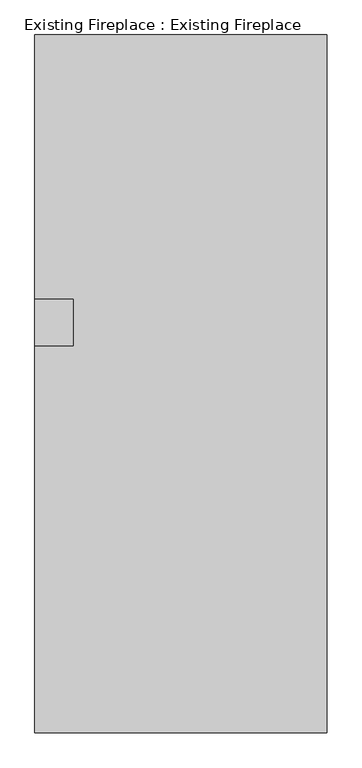
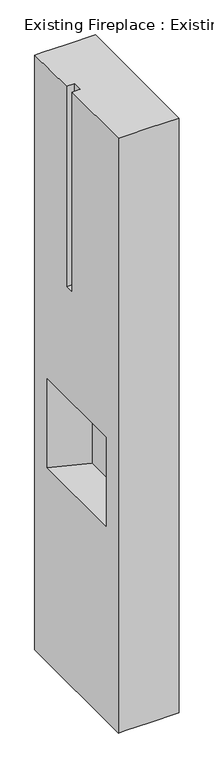
"""IFC4 building model written with IfcOpenShell, lengths in millimetres: proxy geometry, Existing Fireplace : Existing Fireplace."""

import ifcopenshell
import ifcopenshell.guid

model = None  # the IFC model being written
_history = None  # IfcOwnerHistory: only IFC2X3 demands one
_inside = {}  # id of a spatial element -> (the spatial element, [elements in it])
_under = {}  # id of a project, library or spatial element -> (it, [spatial elements below it])
_declared = {}  # id of a project -> (the project, [libraries it declares])
_typed = {}  # id of a type object -> (the type object, [elements of that type])
_made_of = {}  # id of a material, layer set ... -> (it, [elements and type objects made of it])


def new_model(schema):
    """Start an empty IFC model of exactly this schema.

    Asked for "IFC4X3", IfcOpenShell would pick the latest addendum, in which some entities
    have other attributes; the version numbers below select the first issue.
    IFC2X3 requires an IfcOwnerHistory on every rooted entity: one is made here for all.
    """
    global model, _history
    if schema == "IFC4X3":
        model = ifcopenshell.file(schema_version=(4, 3, 0, 0))
    else:
        model = ifcopenshell.file(schema=schema)
    _inside.clear()
    _under.clear()
    _declared.clear()
    _typed.clear()
    _made_of.clear()
    _history = None
    if model.schema == "IFC2X3":
        org = make("IfcOrganization", Name="unknown")
        user = make(
            "IfcPersonAndOrganization",
            ThePerson=make("IfcPerson", FamilyName="unknown"),
            TheOrganization=org,
        )
        app = make(
            "IfcApplication",
            ApplicationDeveloper=org,
            Version="unknown",
            ApplicationFullName="unknown",
            ApplicationIdentifier="unknown",
        )
        _history = make(
            "IfcOwnerHistory",
            OwningUser=user,
            OwningApplication=app,
            ChangeAction="ADDED",
            CreationDate=0,
        )
    return model


def make(cls, **values):
    """One entity of the class cls with the attributes given. An attribute that is None is left unset."""
    return model.create_entity(
        cls, **{name: value for name, value in values.items() if value is not None}
    )


def rooted(cls, **values):
    """An entity with a GlobalId (a new one), such as an element, a storey or a relation."""
    return make(cls, GlobalId=ifcopenshell.guid.new(), OwnerHistory=_history, **values)


def si_unit(unit_type, name, prefix=None):
    """IfcSIUnit, for example si_unit("LENGTHUNIT", "METRE", prefix="MILLI")."""
    return make("IfcSIUnit", UnitType=unit_type, Prefix=prefix, Name=name)


def assignment(units):
    """IfcUnitAssignment: the units of a project."""
    return None if units is None else make("IfcUnitAssignment", Units=units)


def point(xyz):
    """IfcCartesianPoint."""
    return None if xyz is None else make("IfcCartesianPoint", Coordinates=xyz)


def direction(xyz):
    """IfcDirection."""
    return None if xyz is None else make("IfcDirection", DirectionRatios=xyz)


def frame(location, z_axis=None, x_axis=None):
    """IfcAxis2Placement3D, a coordinate frame: its origin and axes. An axis left out is left unset."""
    return make(
        "IfcAxis2Placement3D",
        Location=point(location),
        Axis=direction(z_axis),
        RefDirection=direction(x_axis),
    )


def origin():
    """The frame at (0, 0, 0) with its axes left unset."""
    return frame((0.0, 0.0, 0.0))


def place(relative_to, where):
    """IfcLocalPlacement: puts the frame where relative to a parent placement (None: the world)."""
    return make(
        "IfcLocalPlacement", PlacementRelTo=relative_to, RelativePlacement=where
    )


def context(
    kind, dimensions, precision=None, world=None, true_north=None, identifier=None
):
    """IfcGeometricRepresentationContext, for example the 3D "Model" context."""
    return make(
        "IfcGeometricRepresentationContext",
        ContextIdentifier=identifier,
        ContextType=kind,
        CoordinateSpaceDimension=dimensions,
        Precision=precision,
        WorldCoordinateSystem=world,
        TrueNorth=true_north,
    )


def project(units=None, contexts=None):
    """IfcProject with its units and contexts."""
    return rooted(
        "IfcProject",
        Name="project",
        RepresentationContexts=contexts,
        UnitsInContext=assignment(units),
    )


def spatial(cls, under=None, at=None, **own):
    """A site, building, storey or space (cls), placed at a placement, below another one or the project."""
    s = rooted(cls, ObjectPlacement=at, **own)
    if under is not None:
        _under.setdefault(under.id(), (under, []))[1].append(s)
    return s


def faces_of(points, faces, orient=None, outer=None):
    """IfcFace entities. A face is a list of loops; a loop is a list of indices into points, from 0.

    orient and outer hold one flag for each loop. By default every Orientation is true, the
    first loop of a face is its IfcFaceOuterBound and the others are IfcFaceBound.
    """
    made = []
    for i, loops in enumerate(faces):
        bounds = []
        for j, loop in enumerate(loops):
            is_outer = j == 0 if outer is None else outer[i][j]
            bounds.append(
                make(
                    "IfcFaceOuterBound" if is_outer else "IfcFaceBound",
                    Bound=make("IfcPolyLoop", Polygon=[points[k] for k in loop]),
                    Orientation=True if orient is None else orient[i][j],
                )
            )
        made.append(make("IfcFace", Bounds=bounds))
    return made


def faceted_brep(points, faces, orient=None, outer=None, voids=None):
    """IfcFacetedBrep: a solid bounded by flat faces; with voids (closed shells), ...WithVoids."""
    shared = [point(p) for p in points]
    hull = make("IfcClosedShell", CfsFaces=faces_of(shared, faces, orient, outer))
    if voids is None:
        return make("IfcFacetedBrep", Outer=hull)
    return make(
        "IfcFacetedBrepWithVoids",
        Outer=hull,
        Voids=[
            make(cls, CfsFaces=faces_of(shared, fs, o, b)) for cls, fs, o, b in voids
        ],
    )


def shape(context_of_items, identifier, shape_type, items):
    """IfcShapeRepresentation: the items that make up one representation, for example the "Body"."""
    return make(
        "IfcShapeRepresentation",
        ContextOfItems=context_of_items,
        RepresentationIdentifier=identifier,
        RepresentationType=shape_type,
        Items=items,
    )


def source(mapping_origin, context_of_items, identifier, shape_type, items):
    """IfcRepresentationMap: a shape defined once, which mapped items show again and again."""
    return make(
        "IfcRepresentationMap",
        MappingOrigin=mapping_origin,
        MappedRepresentation=shape(context_of_items, identifier, shape_type, items),
    )


def transform(
    local_origin,
    x_axis=None,
    y_axis=None,
    z_axis=None,
    scale=None,
    scale2=None,
    scale3=None,
    uniform=True,
):
    """IfcCartesianTransformationOperator3D, or its non-uniform kind. x_axis, y_axis, z_axis: its Axis1, 2, 3."""
    if uniform:
        return make(
            "IfcCartesianTransformationOperator3D",
            Axis1=direction(x_axis),
            Axis2=direction(y_axis),
            LocalOrigin=point(local_origin),
            Scale=scale,
            Axis3=direction(z_axis),
        )
    return make(
        "IfcCartesianTransformationOperator3DnonUniform",
        Axis1=direction(x_axis),
        Axis2=direction(y_axis),
        LocalOrigin=point(local_origin),
        Scale=scale,
        Axis3=direction(z_axis),
        Scale2=scale2,
        Scale3=scale3,
    )


def mapped(mapping_source, mapping_target):
    """IfcMappedItem: shows the shape of a source again, moved by a transform."""
    return make(
        "IfcMappedItem", MappingSource=mapping_source, MappingTarget=mapping_target
    )


def made_of(thing, what):
    """Note that an element or type object is made of a material, layer set ...; save() writes the relation."""
    if what is not None:
        _made_of.setdefault(what.id(), (what, []))[1].append(thing)
    return thing


def element(
    cls,
    number,
    at=None,
    inside=None,
    cuts=None,
    type_object=None,
    material=None,
    context=None,
    identifier="Body",
    shape_type=None,
    held_by="IfcProductDefinitionShape",
    body=None,
    shapes=None,
    **own,
):
    """One element of the class cls, such as IfcWall. Its Tag is "e" and its number.

    at: its placement. inside: the storey or other place that contains it. cuts: it is an
    opening in that element (IfcRelVoidsElement). A single representation is given by context,
    identifier, shape_type and body (its items); several are given by shapes. held_by: the class
    of the entity that holds the representations. save() writes the other relations.
    """
    e = rooted(cls, Tag="e%d" % number, ObjectPlacement=at, **own)
    if body is not None:
        shapes = [shape(context, identifier, shape_type, body)]
    if shapes is not None:
        e.Representation = make(held_by, Representations=shapes)
    if inside is not None:
        _inside.setdefault(inside.id(), (inside, []))[1].append(e)
    if cuts is not None:
        rooted(
            "IfcRelVoidsElement", RelatingBuildingElement=cuts, RelatedOpeningElement=e
        )
    if type_object is not None:
        _typed.setdefault(type_object.id(), (type_object, []))[1].append(e)
    return made_of(e, material)


def aggregate(whole, parts):
    """IfcRelAggregates: a whole, such as a stair, and the parts it consists of."""
    return rooted("IfcRelAggregates", RelatingObject=whole, RelatedObjects=parts)


def save(model, path):
    """Write the relations noted so far, then the file.

    IfcRelAggregates (storeys below a building ...), IfcRelContainedInSpatialStructure (elements
    in a storey), IfcRelDefinesByType, IfcRelAssociatesMaterial and IfcRelDeclares: one each for
    every whole, place, type object, material and project.
    """
    for whole, parts in _under.values():
        aggregate(whole, parts)
    for where, things in _inside.values():
        rooted(
            "IfcRelContainedInSpatialStructure",
            RelatedElements=things,
            RelatingStructure=where,
        )
    for kind, things in _typed.values():
        rooted("IfcRelDefinesByType", RelatedObjects=things, RelatingType=kind)
    for what, things in _made_of.values():
        rooted("IfcRelAssociatesMaterial", RelatedObjects=things, RelatingMaterial=what)
    for by, libraries in _declared.values():
        rooted("IfcRelDeclares", RelatingContext=by, RelatedDefinitions=libraries)
    model.write(path)


def existing_fireplace_existing_fireplace_063a625f(model_context):
    return source(origin(), model_context, "Body", "Brep", [
        faceted_brep([(4450.2196932, 434.2888758, 5486.4), (4069.2196932, 434.2888758, 5486.4), (3764.4196932, 434.2888758, 5486.4), (3662.8196932, 434.2888758, 5486.4), (3662.8196932, -276.9111242, 5486.4), (3767.2567114, -276.9111242, 5486.4), (3767.2567114, -403.9111242, 5486.4), (3662.8196932, -403.9111242, 5486.4), (3662.8196932, -1445.3111242, 5486.4), (3764.4196932, -1445.3111242, 5486.4), (4069.2196932, -1445.3111242, 5486.4), (4450.2196932, -1445.3111242, 5486.4), (4450.2196932, 434.2888758, -2667.0), (4450.2196932, -1445.3111242, -2667.0), (4069.2196932, -1445.3111242, -2667.0), (3764.4196932, -1445.3111242, -2667.0), (3662.8196932, -1445.3111242, -2667.0), (3662.8196932, 434.2888758, -2667.0), (3764.4196932, 434.2888758, -2667.0), (4069.2196932, 434.2888758, -2667.0), (3662.8196932, -403.9111242, 2743.2), (3662.8196932, -276.9111242, 2743.2), (3662.8196932, 154.8888758, 0.0), (3662.8196932, 154.8888758, 1219.2), (3662.8196932, -1165.9111242, 1219.2), (3662.8196932, -1165.9111242, 0.0), (4145.4196932, -20.7631592, 1219.2), (4145.4196932, -990.2590891, 1219.2), (4145.4196932, -990.2590891, 0.0), (4145.4196932, -20.7631592, 0.0), (3767.2567114, -403.9111242, 2743.2), (3767.2567114, -276.9111242, 2743.2)], [[[0, 1, 2, 3, 4, 5, 6, 7, 8, 9, 10, 11]], [[12, 13, 14, 15, 16, 17, 18, 19]], [[3, 2, 1, 0, 12, 19, 18, 17]], [[3, 17, 16, 8, 7, 20, 21, 4], [22, 23, 24, 25]], [[11, 10, 9, 8, 16, 15, 14, 13]], [[0, 11, 13, 12]], [[24, 23, 26, 27]], [[25, 24, 27, 28]], [[27, 26, 29, 28]], [[23, 22, 29, 26]], [[22, 25, 28, 29]], [[6, 30, 20, 7]], [[31, 5, 4, 21]], [[30, 31, 21, 20]], [[30, 6, 5, 31]]]),
    ])


if __name__ == "__main__":
    model = new_model("IFC4")
    model_context = context("Model", 3, world=origin())
    ifc_project = project(units=[si_unit("LENGTHUNIT", "METRE", prefix="MILLI")], contexts=[model_context])
    site = spatial("IfcSite", under=ifc_project)
    building = spatial("IfcBuilding", under=site)
    placement = place(None, origin())
    existing_fireplace_existing_fireplace_shape = existing_fireplace_existing_fireplace_063a625f(model_context)
    element("IfcBuildingElementProxy", 1, Name="Existing Fireplace : Existing Fireplace", ObjectType="Existing Fireplace : Existing Fireplace", at=placement, inside=building, context=model_context, shape_type="MappedRepresentation", body=[
        mapped(existing_fireplace_existing_fireplace_shape, transform((0.0, 0.0, 0.0), x_axis=(1.0, 0.0, 0.0), y_axis=(0.0, 1.0, 0.0), z_axis=(0.0, 0.0, 1.0))),
    ])
    save(model, "model.ifc")
